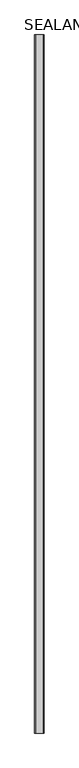
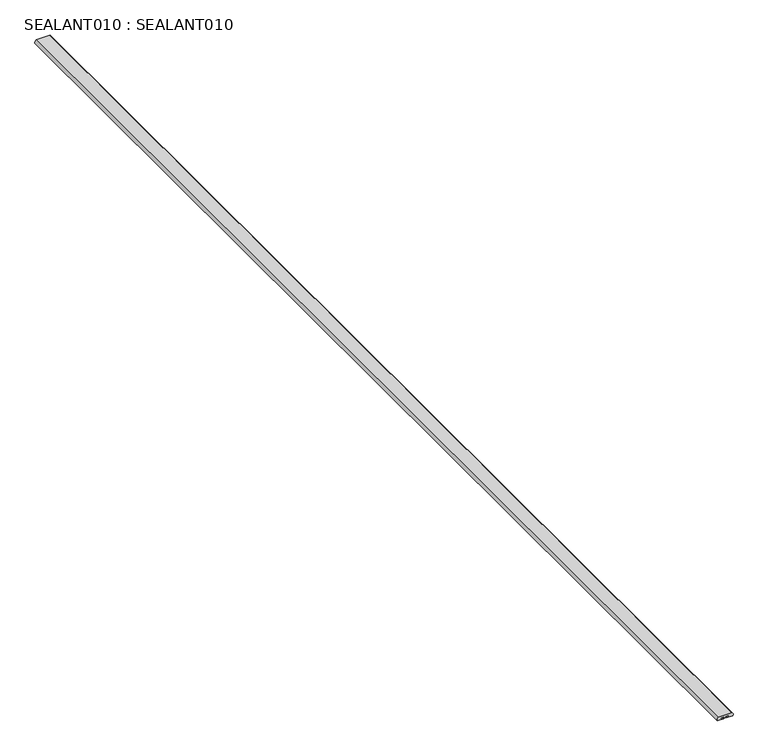
"""IFC4 building model written with IfcOpenShell, lengths in millimetres: proxy geometry, SEALANT010 : SEALANT010."""

from ifc_helpers import new_model, si_unit, point, frame, frame_2d, origin, place, context, project, spatial, polyline, circle_curve, trimmed, segment, composite_curve, outline, extrude, source, transform, mapped, element, save


def sealant010_sealant010_45f8f321(model_context):
    return source(origin(), model_context, "Body", "SweptSolid", [
        extrude(outline(composite_curve([segment(polyline([(42584.5106533, 5991.4047833), (42584.5106533, 5968.0541999)]), True, "CONTINUOUS"), segment(trimmed(circle_curve(frame_2d((42580.2506213, 5971.79781)), 5.6711982), [point((42584.5106533, 5968.0541999))], [point((42578.8995464, 5966.2898988))], False, "CARTESIAN"), True, "CONTINUOUS"), segment(polyline([(42578.8995464, 5966.2898988), (42578.8995464, 5977.3107075), (42579.6987049, 5977.3107075), (42579.6987049, 5972.2671879), (42580.5349921, 5972.2779845), (42582.1288635, 5973.5166866), (42582.1288635, 5978.3957686), (42580.1167322, 5978.792004), (42580.1167322, 5980.039109), (42581.7061629, 5980.039109), (42582.1023984, 5985.3247911), (42580.508527, 5986.5634932), (42579.6987049, 5986.5634932), (42579.6987049, 5981.517626), (42578.8995464, 5981.517626), (42578.8995464, 5993.0234363)]), True, "CONTINUOUS"), segment(trimmed(circle_curve(frame_2d((42580.8909505, 5989.391838)), 4.1417625), [point((42578.8995464, 5993.0234363))], [point((42584.5106533, 5991.4047833))], False, "CARTESIAN"), True, "CONTINUOUS")], self_intersect=False)), frame((0.0, -1052.8906574, 0.0), z_axis=(0.0, 1.0, 0.0), x_axis=(0.0, 0.0, 1.0)), (0.0, 0.0, 1.0), 1999.85),
    ])


if __name__ == "__main__":
    model = new_model("IFC4")
    model_context = context("Model", 3, world=origin())
    ifc_project = project(units=[si_unit("LENGTHUNIT", "METRE", prefix="MILLI")], contexts=[model_context])
    site = spatial("IfcSite", under=ifc_project)
    building = spatial("IfcBuilding", under=site)
    placement = place(None, origin())
    sealant010_sealant010_shape = sealant010_sealant010_45f8f321(model_context)
    element("IfcBuildingElementProxy", 1, Name="SEALANT010 : SEALANT010", ObjectType="SEALANT010 : SEALANT010", at=placement, inside=building, context=model_context, shape_type="MappedRepresentation", body=[
        mapped(sealant010_sealant010_shape, transform((0.0, 0.0, 0.0), x_axis=(1.0, 0.0, 0.0), y_axis=(0.0, 1.0, 0.0), z_axis=(0.0, 0.0, 1.0))),
    ])
    save(model, "model.ifc")

# Revit data of these elements
# Type "SEALANT010 : SEALANT010"
#   NameOverride = "SEALANT010"
# Element 1 (IfcBuildingElementProxy, "SEALANT010 : SEALANT010")
#   Materials on its faces: "3/8\" BEAD NON-SINKING BUTYL SEALANT"
# Materials
#   "3/8\" BEAD NON-SINKING BUTYL SEALANT": class "Unassigned", colour RGB 140 208 103, transparency 0
